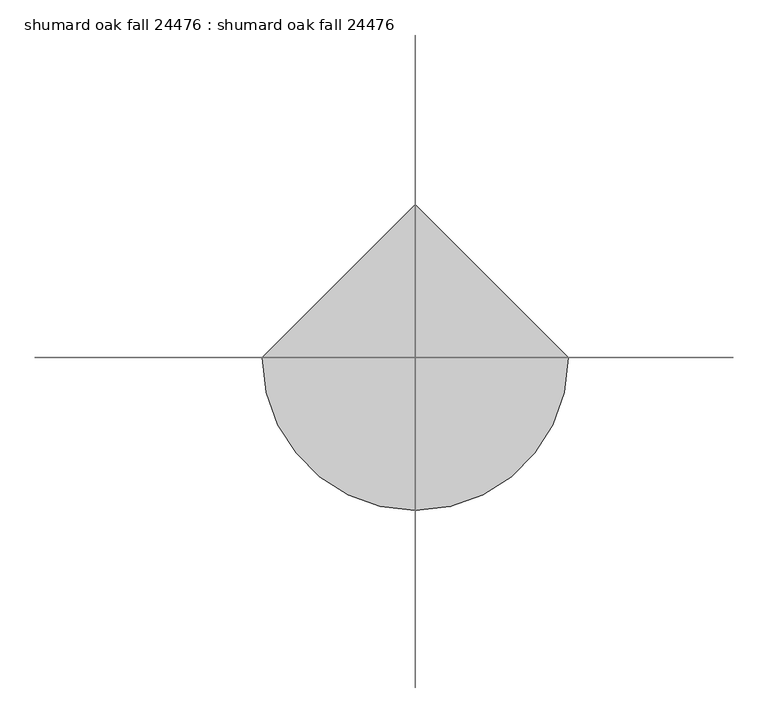
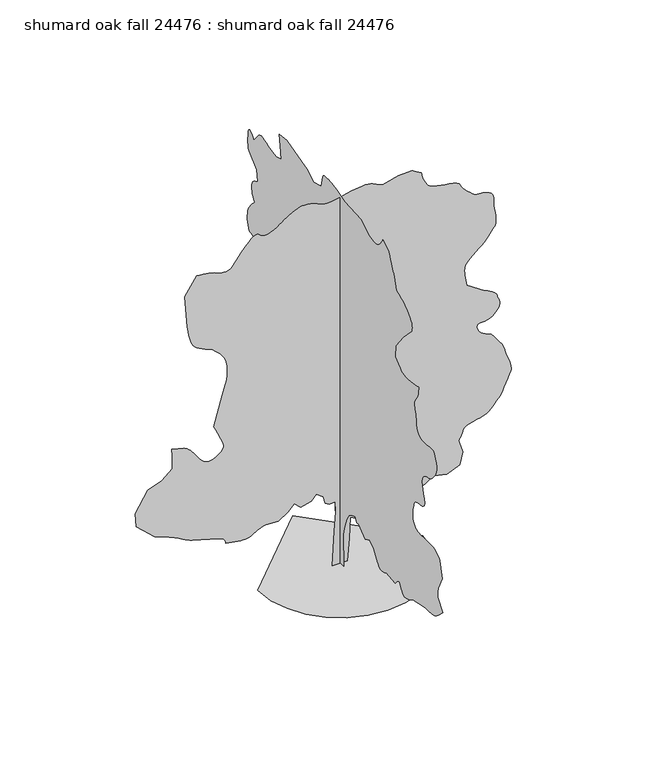
"""IFC4 building model written with IfcOpenShell, lengths in millimetres: proxy geometry, shumard oak fall 24476 : shumard oak fall 24476."""

from ifc_helpers import new_model, si_unit, origin, place, context, project, spatial, triangles, source, transform, mapped, element, save


def shumard_oak_fall_24476_shumard_oak_fall_24476_f3c00e57(model_context):
    return source(origin(), model_context, "Body", "Tessellation", [
        triangles([(-0.002261, 219.4990839, 0.0114695), (-0.002261, -202.1468545, 0.0114695), (-0.002261, -165.4815053, 1044.9594), (-0.002261, -238.8111863, 1356.611816), (-0.002261, -348.8074883, 1649.9305401), (-0.002261, -477.1331583, 1851.5859638), (-0.002261, -623.7925203, 1943.2492641), (-0.002261, -807.1167229, 2016.5789452), (-0.002261, -880.4464039, 1851.5859638), (-0.002261, -1008.7746174, 1888.2507317), (-0.002261, -1155.4339794, 1741.5913696), (-0.002261, -1357.0894032, 1613.2657722), (-0.002261, -1595.4095947, 1723.2602211), (-0.002261, -1815.3986378, 1576.6008591), (-0.002261, -1962.0604706, 1319.9470482), (-0.002261, -1997.5492928, 1269.2765945), (-0.002261, -2033.8382114, 1221.0141335), (-0.002261, -2071.73241, 1177.5624252), (-0.002261, -2112.0319851, 1141.3243029), (-0.002261, -2155.5370331, 1114.7076862), (-0.002261, -2203.0527374, 1100.1179518), (-0.002261, -2255.3767239, 1099.955389), (-0.002261, -2305.5645035, 1108.8834778), (-0.002261, -2347.093364, 1119.7317982), (-0.002261, -2381.4062405, 1132.1853985), (-0.002261, -2409.948103, 1145.9216967), (-0.002261, -2434.1594158, 1160.6206541), (-0.002261, -2455.4852943, 1175.9596888), (-0.002261, -2475.3657669, 1191.618762), (-0.002261, -2952.0087662, 1136.622773), (-0.002261, -2998.9986305, 1190.8694618), (-0.002261, -3044.9978577, 1240.6280525), (-0.002261, -3089.0922592, 1281.4101562), (-0.002261, -3130.3164871, 1308.7227333), (-0.002261, -3167.6796135, 1318.0750694), (-0.002261, -3200.2171623, 1304.9813919), (-0.002261, -3226.9884933, 1264.9485157), (-0.002261, -3253.8871422, 1207.3845148), (-0.002261, -3287.1865631, 1147.8978115), (-0.002261, -3326.5565437, 1091.299086), (-0.002261, -3371.7430298, 1042.3940042), (-0.002261, -3422.3396507, 1005.9958626), (-0.002261, -3478.092643, 986.9154139), (-0.002261, -3538.6462143, 989.9608675), (-0.002261, -3599.3521019, 1007.8145016), (-0.002261, -3656.2224678, 1029.5136858), (-0.002261, -3709.8927383, 1054.4208864), (-0.002261, -3760.9974678, 1081.8909393), (-0.002261, -3810.1717918, 1111.2888542), (-0.002261, -3858.0505554, 1141.9669235), (-0.002261, -3905.294474, 1173.2876135), (-0.002261, -4565.2617485, 1301.6132835), (-0.002261, -4647.5828865, 1301.7733028), (-0.002261, -4728.7613617, 1302.8960541), (-0.002261, -4807.7042175, 1305.9439785), (-0.002261, -4883.2693726, 1311.8748665), (-0.002261, -4954.3638702, 1321.6563915), (-0.002261, -5019.8447571, 1336.2461987), (-0.002261, -5078.5696609, 1356.611816), (-0.002261, -5135.1603928, 1386.0605999), (-0.002261, -5194.6474594, 1426.09086), (-0.002261, -5256.5471695, 1474.9426746), (-0.002261, -5320.3769943, 1530.8479832), (-0.002261, -5385.6294067, 1592.0465733), (-0.002261, -5451.8474579, 1656.7708202), (-0.002261, -5518.5474564, 1723.2602211), (-0.002261, -5261.9061447, 2016.5789452), (-0.002261, -5254.2612625, 2071.5216671), (-0.002261, -5247.8854889, 2126.1442051), (-0.002261, -5244.1008362, 2180.1268112), (-0.002261, -5244.1519958, 2233.1466854), (-0.002261, -5249.3336563, 2284.8837891), (-0.002261, -5260.9410873, 2335.0182289), (-0.002261, -5280.2195618, 2383.2273502), (-0.002261, -5481.8956238, 2804.8665848), (-0.002261, -5353.5493881, 3318.1744972), (-0.002261, -5343.5162796, 3332.34776), (-0.002261, -5313.5698517, 3368.644091), (-0.002261, -5264.0908951, 3417.7422569), (-0.002261, -5195.3584625, 3470.3963104), (-0.002261, -5107.7033478, 3517.2594383), (-0.002261, -5001.4551819, 3549.0601135), (-0.002261, -4876.9191788, 3556.5023918), (-0.002261, -4738.1593346, 3550.7364647), (-0.002261, -4595.2590454, 3548.4758469), (-0.002261, -4457.4642586, 3548.8060593), (-0.002261, -4334.0967888, 3550.7364647), (-0.002261, -4234.4781601, 3553.3020058), (-0.002261, -4167.8793182, 3555.5370438), (-0.002261, -4143.6223686, 3556.5023918), (-0.002261, -4129.3985275, 3566.1797081), (-0.002261, -4092.7461136, 3593.4847275), (-0.002261, -4042.6067322, 3635.877198), (-0.002261, -3987.9714043, 3690.7665802), (-0.002261, -3937.857312, 3755.5873329), (-0.002261, -3901.1798996, 3827.7992043), (-0.002261, -3886.9557678, 3904.8119453), (-0.002261, -3889.6480453, 3981.7738174), (-0.002261, -3897.1159035, 4055.8655159), (-0.002261, -3908.5965981, 4127.5442802), (-0.002261, -3923.3032585, 4197.2923485), (-0.002261, -3940.4225624, 4265.5928307), (-0.002261, -3959.1170609, 4332.9282555), (-0.002261, -3978.6243004, 4399.7808609), (-0.002261, -3994.6515198, 4419.3642586), (-0.002261, -4012.6094353, 4438.4398384), (-0.002261, -4034.4278709, 4456.5497795), (-0.002261, -4062.0122337, 4473.2377144), (-0.002261, -4097.2673492, 4487.969664), (-0.002261, -4142.1744919, 4500.3392578), (-0.002261, -4198.6131981, 4509.7880997), (-0.002261, -4266.863102, 4515.5540268), (-0.002261, -4340.573719, 4522.2850113), (-0.002261, -4411.7190857, 4537.6773857), (-0.002261, -4472.2723663, 4569.4271919), (-0.002261, -4514.2331772, 4625.2310532), (-0.002261, -4529.5493935, 4712.7847206), (-0.002261, -4510.270919, 4839.758947), (-0.002261, -4470.7739113, 4983.3196609), (-0.002261, -4434.4772896, 5115.0185989), (-0.002261, -4406.8420578, 5234.2206253), (-0.002261, -4393.3295105, 5340.2397354), (-0.002261, -4399.3744904, 5432.492244), (-0.002261, -4430.4132935, 5510.3177261), (-0.002261, -4491.9319221, 5573.0557571), (-0.002261, -4567.3444702, 5616.9978424), (-0.002261, -4637.3213036, 5643.9473602), (-0.002261, -4703.1074043, 5661.5747726), (-0.002261, -4766.0230408, 5677.6022827), (-0.002261, -4827.313195, 5699.725351), (-0.002261, -4888.2981354, 5735.6661804), (-0.002261, -4950.2490051, 5793.0446548), (-0.002261, -5013.3678268, 5866.0698486), (-0.002261, -5073.5908951, 5943.8953308), (-0.002261, -5125.8132889, 6026.8263153), (-0.002261, -5164.8783463, 6115.2435928), (-0.002261, -5185.6811462, 6209.4012177), (-0.002261, -5183.0650269, 6309.6799805), (-0.002261, -5151.8989059, 6416.3600967), (-0.002261, -5114.282016, 6517.2737045), (-0.002261, -5088.8312439, 6599.5698441), (-0.002261, -5065.3105865, 6662.6380875), (-0.002261, -5033.4590424, 6705.8180099), (-0.002261, -4983.0150284, 6728.499765), (-0.002261, -4903.6908005, 6729.9985107), (-0.002261, -4785.2506462, 6709.6788208), (-0.002261, -4644.7382927, 6687.2249588), (-0.002261, -4509.6866524, 6682.729303), (-0.002261, -4385.5061508, 6696.2168518), (-0.002261, -4277.7086609, 6727.6364456), (-0.002261, -4191.7298973, 6777.0142456), (-0.002261, -4132.9797043, 6844.3746689), (-0.002261, -4106.9449562, 6929.6677185), (-0.002261, -4098.029512, 7020.7516937), (-0.002261, -4087.1836624, 7106.0447433), (-0.002261, -4074.7123306, 7186.5375046), (-0.002261, -4060.9963074, 7263.169455), (-0.002261, -4046.2896469, 7336.9306503), (-0.002261, -4030.9481415, 7408.761731), (-0.002261, -4015.3017128, 7479.6277542), (-0.002261, -4000.0616547, 7530.732193), (-0.002261, -3987.71735, 7581.9895294), (-0.002261, -3981.1389725, 7633.5764969), (-0.002261, -3983.2216942, 7685.6215759), (-0.002261, -3996.8612686, 7738.3264984), (-0.002261, -4024.9028709, 7791.8185822), (-0.002261, -4070.2925423, 7846.2763046), (-0.002261, -4118.8067322, 7913.1036209), (-0.002261, -4155.4841446, 7996.8979248), (-0.002261, -4181.8746849, 8087.7534256), (-0.002261, -4199.6294151, 8175.7387527), (-0.002261, -4210.3226578, 8250.8719574), (-0.002261, -4215.5551872, 8303.2722473), (-0.002261, -4216.952195, 8322.9315125), (-0.002261, -4189.9012299, 8316.8865326), (-0.002261, -4117.3332756, 8301.5450272), (-0.002261, -4012.0251686, 8281.0724396), (-0.002261, -3886.8543205, 8259.6603745), (-0.002261, -3754.6219849, 8241.4231155), (-0.002261, -3628.1808655, 8230.5772659), (-0.002261, -3520.3075081, 8231.2632706), (-0.002261, -3429.2485313, 8247.1384644), (-0.002261, -3343.9301926, 8277.4401031), (-0.002261, -3263.437722, 8319.7822861), (-0.002261, -3186.8057716, 8371.7250458), (-0.002261, -3113.0442856, 8430.9068985), (-0.002261, -3041.213205, 8494.8640411), (-0.002261, -2970.3474724, 8561.259407), (-0.002261, -2988.6861786, 8946.2469543), (-0.002261, -3391.9868523, 9459.5545761), (-0.002261, -3850.3036446, 9936.1842041), (-0.002261, -3857.4662888, 9995.2898987), (-0.002261, -3860.4634895, 10055.5385468), (-0.002261, -3855.1042236, 10118.0231049), (-0.002261, -3837.2480461, 10183.8597839), (-0.002261, -3802.7295135, 10254.1927002), (-0.002261, -3747.3576027, 10330.1380646), (-0.002261, -3666.9668701, 10412.8399933), (-0.002261, -3572.6822182, 10492.2909576), (-0.002261, -3478.4228554, 10559.2705902), (-0.002261, -3384.1382034, 10615.8113251), (-0.002261, -3289.8535515, 10664.0200104), (-0.002261, -3195.5688995, 10705.9814026), (-0.002261, -3101.2842476, 10743.77677), (-0.002261, -3006.9995956, 10779.4629639), (-0.002261, -2979.491391, 10873.4944336), (-0.002261, -2951.8055809, 10965.8992584), (-0.002261, -2923.7892677, 11055.1042786), (-0.002261, -2895.2904259, 11139.5072662), (-0.002261, -2866.1823189, 11217.4862274), (-0.002261, -2836.2356003, 11287.4366089), (-0.002261, -2805.3494041, 11347.7875763), (-0.002261, -2771.0846352, 11413.5730957), (-0.002261, -2733.3151382, 11494.7518616), (-0.002261, -2695.1895584, 11582.0511841), (-0.002261, -2659.9853119, 11666.1251221), (-0.002261, -2630.8516251, 11737.6765686), (-0.002261, -2611.0141731, 11787.4351593), (-0.002261, -2603.698922, 11806.1037872), (-0.002261, -2292.0441078, 11989.4158539), (-0.002261, -2276.0623798, 11957.8177826), (-0.002261, -2258.4779881, 11925.2813965), (-0.002261, -2237.6856525, 11890.8137329), (-0.002261, -2212.0850349, 11853.4497345), (-0.002261, -2180.0708553, 11812.2255066), (-0.002261, -2140.0379791, 11766.2259888), (-0.002261, -2090.3862133, 11714.4361267), (-0.002261, -2030.5793987, 11669.5795624), (-0.002261, -1962.1138103, 11643.0369965), (-0.002261, -1886.4320927, 11631.6830383), (-0.002261, -1804.9770355, 11632.5469391), (-0.002261, -1719.1937542, 11642.5544678), (-0.002261, -1630.5250385, 11658.6325562), (-0.002261, -1540.413533, 11677.7581329), (-0.002261, -1137.1002874, 11952.7378601), (-0.002261, -257.1441153, 12007.7542694), (-0.002261, -143.4615103, 12039.0221283), (-0.002261, -31.2221381, 12069.3237671), (-0.002261, 78.1307869, 12097.6952911), (-0.002261, 183.1547906, 12123.1972229), (-0.002261, 282.4069083, 12144.8377625), (-0.002261, 374.4436778, 12161.678595), (-0.002261, 457.8190392, 12172.7523376), (-0.002261, 540.0209258, 12181.1855438), (-0.002261, 626.0734131, 12188.6781097), (-0.002261, 710.8406954, 12191.9802338), (-0.002261, 789.1944883, 12187.9165283), (-0.002261, 856.001457, 12173.286026), (-0.002261, 906.1358969, 12144.8377625), (-0.002261, 934.464473, 12099.3975128), (-0.002261, 1026.1253025, 11732.7745422), (-0.002261, 1429.4386208, 11622.7673035), (-0.002261, 1796.0870258, 11842.7562012), (-0.002261, 2254.3987312, 11952.7378601), (-0.002261, 2859.3748856, 12136.0755066), (-0.002261, 3262.6755592, 12081.0846771), (-0.002261, 3226.023436, 11732.7745422), (-0.002261, 3152.6939003, 11329.4491608), (-0.002261, 3446.0126244, 11237.7803375), (-0.002261, 3739.3313484, 11292.771167), (-0.002261, 3852.7421585, 11335.3918213), (-0.002261, 3963.1048988, 11374.2801453), (-0.002261, 4067.3717903, 11405.8258942), (-0.002261, 4162.5200523, 11426.2990631), (-0.002261, 4245.476326, 11432.0138306), (-0.002261, 4313.1925415, 11419.2878632), (-0.002261, 4362.6209198, 11384.4399902), (-0.002261, 4637.600647, 11054.4682709), (-0.002261, 4700.0846237, 11127.5184631), (-0.002261, 4760.3332718, 11191.1203949), (-0.002261, 4816.0609749, 11235.7990631), (-0.002261, 4865.082692, 11252.1062073), (-0.002261, 4905.1133881, 11230.5668243), (-0.002261, 4933.9168625, 11161.7326538), (-0.002261, 4949.2583679, 11036.1298553), (-0.002261, 4953.90634, 10896.6337189), (-0.002261, 4952.7889664, 10788.8868073), (-0.002261, 4946.870723, 10707.5813049), (-0.002261, 4937.0660889, 10647.4593933), (-0.002261, 4924.416861, 10603.2132568), (-0.002261, 4909.8119385, 10569.5327545), (-0.002261, 4894.2675385, 10541.1612305), (-0.002261, 4472.6281586, 10192.8255157), (-0.002261, 4435.9504555, 9807.8641296), (-0.002261, 4494.5989105, 9783.9632629), (-0.002261, 4551.4439873, 9758.1566986), (-0.002261, 4604.7840454, 9728.4893234), (-0.002261, 4652.8407051, 9693.0560211), (-0.002261, 4693.8361679, 9649.9272583), (-0.002261, 4726.0179245, 9597.1711761), (-0.002261, 4747.6078857, 9532.8588226), (-0.002261, 4755.837616, 9462.1706955), (-0.002261, 4750.6050865, 9391.4569885), (-0.002261, 4734.1459167, 9320.7438629), (-0.002261, 4708.6951447, 9250.0301559), (-0.002261, 4676.5133881, 9179.316449), (-0.002261, 4639.8612648, 9108.6033234), (-0.002261, 4600.9485237, 9037.8896164), (-0.002261, 4659.6225586, 8978.9362381), (-0.002261, 4716.8740059, 8919.8305435), (-0.002261, 4771.2299904, 8860.3946365), (-0.002261, 4821.2679245, 8800.4762009), (-0.002261, 4865.5146423, 8739.9229202), (-0.002261, 4902.547847, 8678.581897), (-0.002261, 4930.919371, 8616.2502365), (-0.002261, 4951.2902206, 8555.5446396), (-0.002261, 4965.8951431, 8498.6742737), (-0.002261, 4975.6741974, 8445.0037125), (-0.002261, 4981.5924408, 8393.8992737), (-0.002261, 4984.6405106, 8344.7249496), (-0.002261, 4985.7578842, 8296.8458954), (-0.002261, 4985.9357803, 8249.6022675), (-0.002261, 4875.9285416, 7937.9445465), (-0.002261, 4824.8999702, 7929.765976), (-0.002261, 4773.9984261, 7919.6817078), (-0.002261, 4723.4526741, 7905.7122116), (-0.002261, 4673.363871, 7886.0017868), (-0.002261, 4623.9354927, 7858.5697403), (-0.002261, 4575.2945663, 7821.5365356), (-0.002261, 4527.618988, 7772.9464783), (-0.002261, 4484.2103004, 7715.2883698), (-0.002261, 4447.5581772, 7652.804393), (-0.002261, 4416.4940849, 7586.332869), (-0.002261, 4389.9256485, 7516.635379), (-0.002261, 4366.7354942, 7444.5246643), (-0.002261, 4345.7806686, 7370.8140472), (-0.002261, 4325.9687965, 7296.3162689), (-0.002261, 4283.0426376, 7237.3628906), (-0.002261, 4241.8948586, 7178.257196), (-0.002261, 4204.2520981, 7118.8212891), (-0.002261, 4171.9180252, 7058.9028534), (-0.002261, 4146.6448586, 6998.3489914), (-0.002261, 4130.1856888, 6936.9829697), (-0.002261, 4124.2930252, 6874.676889), (-0.002261, 4142.6317314, 6379.682103), (-0.002261, 4185.5575996, 6375.3643433), (-0.002261, 4226.7056694, 6368.6333588), (-0.002261, 4264.3484299, 6357.076506), (-0.002261, 4296.6825027, 6338.3311386), (-0.002261, 4321.9553787, 6309.9340347), (-0.002261, 4338.4145485, 6269.5481277), (-0.002261, 4344.2819229, 6214.7096146), (-0.002261, 4342.6817299, 6151.3111588), (-0.002261, 4338.2113632, 6086.9732254), (-0.002261, 4331.3027733, 6021.822551), (-0.002261, 4322.4887764, 5956.0108704), (-0.002261, 4312.2271935, 5889.7428223), (-0.002261, 4301.0005531, 5823.1439804), (-0.002261, 4289.2910934, 5756.3928223), (-0.002261, 4270.9523872, 5389.7442719), (-0.002261, 4619.2875206, 5408.0832687), (-0.002261, 5004.2491974, 5481.4130951), (-0.002261, 5086.1895447, 5453.6758347), (-0.002261, 5164.7516098, 5424.4915695), (-0.002261, 5236.6082703, 5392.4115509), (-0.002261, 5298.3300842, 5356.0131912), (-0.002261, 5346.5899292, 5313.8494858), (-0.002261, 5378.009523, 5264.4716858), (-0.002261, 5389.2361633, 5206.4072067), (-0.002261, 5386.0357773, 5132.8744858), (-0.002261, 5377.0444656, 5040.0882889), (-0.002261, 5363.2778641, 4931.2751633), (-0.002261, 5345.6248718, 4809.634623), (-0.002261, 5325.1017059, 4678.3676353), (-0.002261, 5302.6478439, 4540.6745865), (-0.002261, 5279.2545044, 4399.7808609), (-0.002261, 5114.2564362, 3959.8027748), (-0.002261, 5024.1375183, 3909.2570229), (-0.002261, 4935.4661865, 3861.7337608), (-0.002261, 4849.6903175, 3820.3063477), (-0.002261, 4768.2327896, 3788.0228531), (-0.002261, 4692.5661873, 3767.9316376), (-0.002261, 4624.0880997, 3763.0801895), (-0.002261, 4564.2711113, 3776.4912895), (-0.002261, 4050.9631989, 3996.4804779), (-0.002261, 3537.6555771, 3831.4824097), (-0.002261, 3171.0070267, 3574.841098), (-0.002261, 2804.3587669, 3024.8557732), (-0.002261, 2768.8748863, 2970.1951561), (-0.002261, 2732.6038445, 2917.4393646), (-0.002261, 2694.7070297, 2868.5190948), (-0.002261, 2654.3972809, 2825.3897507), (-0.002261, 2610.887146, 2789.9570297), (-0.002261, 2563.3891731, 2764.1504654), (-0.002261, 2511.0525421, 2749.8757553), (-0.002261, 2458.8327644, 2745.1260452), (-0.002261, 2409.8236919, 2745.4815468), (-0.002261, 2360.4918194, 2749.3932266), (-0.002261, 2307.3119259, 2755.2097321), (-0.002261, 2246.7558838, 2761.3564499), (-0.002261, 2175.2957108, 2766.2334778), (-0.002261, 2089.4057499, 2768.2144615), (-0.002261, 1997.2622463, 2761.2550026), (-0.002261, 1908.966909, 2741.798632), (-0.002261, 1823.8796608, 2711.9283623), (-0.002261, 1741.357663, 2673.7013351), (-0.002261, 1660.7585129, 2629.251432), (-0.002261, 1581.4421333, 2580.6105057), (-0.002261, 1502.7683018, 2529.8868576), (-0.002261, 1392.7737076, 2218.2343689), (-0.002261, 1081.123835, 1869.9195831), (-0.002261, 1038.0988449, 1823.313271), (-0.002261, 988.3377834, 1777.6695454), (-0.002261, 932.9658726, 1732.8259163), (-0.002261, 873.1057909, 1688.6248352), (-0.002261, 809.8776735, 1644.9064281), (-0.002261, 744.404199, 1601.5055889), (-0.002261, 677.8105894, 1558.2672398), (-0.002261, 567.8161042, 1943.2492641), (-0.002261, 384.4893582, 2199.9032204), (-0.002261, 311.1621843, 2034.9100937), (-0.002261, 256.16367, 1778.2562828), (-0.002261, 237.8317585, 1319.9470482), (-0.002261, 201.1664093, 678.3109949), (227.1495435, 0.0005814, 0.0290322), (-249.4926201, 0.0005814, 0.0290322), (-176.1637021, 0.0005159, 1099.9731932), (-139.4986073, 0.0004774, 1741.6091011), (-157.8310275, 0.0004578, 2071.5927383), (-341.1570105, 0.0004589, 2053.2615898), (-469.4826805, 0.0004547, 2126.5912708), (-524.4786695, 0.0004403, 2364.9114624), (-744.470256, 0.0004316, 2511.5708244), (-891.1296181, 0.0004414, 2346.5778431), (-1221.1106392, 0.000447, 2254.9170135), (-1422.7685337, 0.0004361, 2438.2411434), (-1624.4239574, 0.000448, 2236.5832489), (-1917.7426815, 0.0004589, 2053.2615898), (-2357.7232384, 0.0004578, 2071.5927383), (-2577.7147522, 0.0004634, 1979.929438), (-2624.9586708, 0.0004655, 1944.816465), (-2672.8377251, 0.0004676, 1911.143811), (-2722.0120491, 0.0004694, 1880.3590622), (-2773.1167786, 0.0004708, 1853.9023922), (-2826.7867584, 0.0004722, 1833.219207), (-2883.6321259, 0.0004729, 1819.7496803), (-2944.3633026, 0.0004732, 1814.9389275), (-3012.0286491, 0.0004732, 1817.0776051), (-3088.3556763, 0.0004729, 1823.0618328), (-3171.8962166, 0.0004722, 1832.2566204), (-3261.2023933, 0.0004715, 1844.0141876), (-3354.8266205, 0.0004708, 1857.6972187), (-3451.3718903, 0.0004697, 1872.662875), (-3549.3394569, 0.000469, 1888.2686085), (-3553.8606926, 0.0004666, 1927.4454323), (-3562.115712, 0.0004641, 1965.9797081), (-3577.7112717, 0.000462, 2003.2338295), (-3604.3811554, 0.0004599, 2038.5626324), (-3645.8085686, 0.0004578, 2071.3260395), (-3705.6508461, 0.0004561, 2100.8815029), (-3787.6420624, 0.0004547, 2126.5912708), (-4594.2684082, 0.0004403, 2364.9114624), (-4660.1306671, 0.0004393, 2385.8106228), (-4730.463002, 0.0004375, 2415.3659409), (-4803.0306656, 0.0004354, 2451.0149277), (-4875.623909, 0.000433, 2490.1916061), (-4945.9562439, 0.0004305, 2530.3313072), (-5011.8185028, 0.0004284, 2568.8757568), (-5070.9241974, 0.0004263, 2603.2419731), (-5134.4749695, 0.0004242, 2636.2617599), (-5213.4178253, 0.0004221, 2672.1773003), (-5305.1878052, 0.0004197, 2710.5057747), (-5407.219368, 0.0004176, 2750.7393654), (-5516.947554, 0.0004151, 2792.446122), (-5631.8062408, 0.0004123, 2835.0926468), (-5749.2298874, 0.0004099, 2878.2217003), (-6317.52892, 0.000378, 3409.8683189), (-6354.1807526, 0.0003518, 3849.846405), (-5969.2187851, 0.0003147, 4473.1359764), (-5529.2409897, 0.0003049, 4638.1340446), (-5199.2448532, 0.0002884, 4913.1140625), (-5199.2448532, 0.0002636, 5334.7534424), (-5217.5832687, 0.0002503, 5554.7423401), (-4832.5963028, 0.0002559, 5463.099678), (-4789.264064, 0.0002576, 5435.1339432), (-4745.0935043, 0.0002594, 5404.4509323), (-4699.3480408, 0.0002615, 5368.3322067), (-4651.1896431, 0.0002639, 5324.0093307), (-4599.8311501, 0.0002674, 5268.8150253), (-4544.4592392, 0.0002716, 5199.9814362), (-4484.2867493, 0.0002765, 5114.7645447), (-4423.3012276, 0.0002818, 5025.254892), (-4364.5513252, 0.0002867, 4946.3120361), (-4305.8264214, 0.0002905, 4879.560878), (-4244.8411903, 0.0002937, 4826.5766121), (-4179.3600128, 0.0002961, 4789.0100098), (-4107.1481415, 0.0002972, 4768.4359749), (-4025.9696663, 0.0002972, 4766.4547005), (-3937.1968872, 0.0002961, 4786.7746811), (-3847.7889725, 0.0002937, 4827.9227509), (-3763.8167725, 0.0002902, 4883.8280594), (-3691.4014252, 0.0002863, 4948.3944672), (-3636.613781, 0.0002825, 5015.5269974), (-3605.5496887, 0.0002786, 5079.1283478), (-3604.3305771, 0.0002755, 5133.1029602), (-3625.9205383, 0.000272, 5191.4720718), (-3658.1020042, 0.0002674, 5270.034137), (-3699.0977577, 0.0002615, 5365.4364532), (-3747.1291283, 0.0002552, 5474.3263184), (-3800.4688957, 0.0002482, 5593.2998703), (-3857.3395523, 0.0002405, 5719.0038254), (-3915.9880074, 0.0002328, 5848.0610641), (-3659.3214066, 0.0001771, 6783.0336456), (-3624.2186073, 0.0001708, 6888.8498611), (-3590.5383957, 0.0001645, 6993.2440704), (-3559.7536469, 0.0001586, 7094.7419449), (-3533.2866577, 0.0001526, 7191.8970612), (-3512.6111755, 0.0001474, 7283.2856689), (-3499.1492065, 0.0001421, 7367.4613449), (-3494.3233383, 0.0001379, 7443.0009201), (-3495.5677391, 0.0001334, 7516.6859573), (-3499.6826042, 0.0001288, 7594.8928116), (-3507.3280678, 0.0001239, 7675.3344131), (-3519.1389748, 0.000119, 7755.7760147), (-3535.7504608, 0.0001145, 7833.9572891), (-3557.8232414, 0.0001099, 7907.6679062), (-3585.9915802, 0.0001061, 7974.6219589), (-3622.2373329, 0.0001022, 8036.9536194), (-3667.1191864, 9.87e-05, 8098.3196411), (-3719.2398422, 9.52e-05, 8158.8735031), (-3777.1264252, 9.14e-05, 8218.7919388), (-3839.3307678, 8.79e-05, 8278.2022659), (-3904.430864, 8.44e-05, 8337.3335403), (-3970.9788368, 8.09e-05, 8396.2869186), (-4076.5918671, 7.84e-05, 8439.5685791), (-4179.4617508, 7.56e-05, 8483.3321869), (-4276.8959198, 7.32e-05, 8528.0870132), (-4366.1768074, 7.04e-05, 8574.2644272), (-4444.5103981, 6.76e-05, 8622.3719559), (-4509.254702, 6.44e-05, 8672.8671295), (-4557.6162849, 6.13e-05, 8726.2574753), (-4595.665416, 5.71e-05, 8797.4537109), (-4630.8443733, 5.15e-05, 8893.9734009), (-4662.4674431, 4.48e-05, 9005.2509109), (-4689.9500679, 3.78e-05, 9120.6938644), (-4712.6068245, 3.12e-05, 9229.7354645), (-4729.828157, 2.59e-05, 9321.7594986), (-4740.9277702, 2.21e-05, 9386.2247498), (-4814.2575966, -3.92e-05, 10412.8399933), (-4447.6090462, -7.32e-05, 10981.1390259), (-4349.6414795, -7.25e-05, 10969.2269623), (-4253.1214989, -7.18e-05, 10956.5009949), (-4159.4719826, -7.07e-05, 10942.1751251), (-4070.1658058, -6.97e-05, 10925.4621918), (-3986.6252655, -6.86e-05, 10905.5238739), (-3910.3238182, -6.72e-05, 10881.5706848), (-3842.658181, -6.55e-05, 10852.8189514), (-3773.849881, -6.37e-05, 10825.0311127), (-3696.4051895, -6.27e-05, 10805.5741608), (-3615.1255577, -6.2e-05, 10796.0491608), (-3534.7854034, -6.23e-05, 10798.0815948), (-3460.2364655, -6.3e-05, 10813.2702026), (-3396.2540337, -6.48e-05, 10843.1916321), (-3347.6639763, -6.76e-05, 10889.4957825), (-3054.3452522, -9.07e-05, 11274.4583313), (-2976.0116615, -9.59e-05, 11364.1447174), (-2898.9227623, -0.0001012, 11449.8185577), (-2824.4246933, -0.0001057, 11527.4917236), (-2753.7618553, -0.0001096, 11593.1260895), (-2688.2300995, -0.0001127, 11642.7312012), (-2629.1244049, -0.0001145, 11672.2724213), (-2577.7147522, -0.0001148, 11677.7837128), (-2536.3434402, -0.0001138, 11663.9915314), (-2502.6707863, -0.0001124, 11641.5382507), (-2470.9233055, -0.000111, 11615.2491577), (-2435.3278038, -0.0001096, 11589.9251221), (-2390.1107964, -0.0001082, 11570.3414337), (-2329.5038853, -0.0001078, 11561.3757019), (-2247.7287895, -0.0001082, 11567.776474), (-2150.0253056, -0.0001099, 11595.5898926), (-2049.7588966, -0.0001124, 11641.9696198), (-1953.3381832, -0.0001159, 11698.6370911), (-1867.1815235, -0.0001194, 11757.2090973), (-1797.6998634, -0.0001225, 11809.3803314), (-1751.3093811, -0.0001246, 11846.7699097), (-1734.4184063, -0.0001257, 11861.0957794), (-1713.7352211, -0.0001264, 11874.3542725), (-1658.7366886, -0.0001285, 11908.7707764), (-1580.0095173, -0.0001313, 11956.3446167), (-1488.1328579, -0.0001344, 12009.0495392), (-1393.6932735, -0.0001372, 12058.8592896), (-1307.269915, -0.0001397, 12097.7720306), (-1239.4444038, -0.0001407, 12117.7615082), (-1175.0935352, -0.0001411, 12122.2065857), (-1095.0303263, -0.0001411, 12119.5648865), (-1003.7428751, -0.0001404, 12109.5829376), (-905.7193525, -0.0001393, 12091.8793671), (-805.4530163, -0.0001379, 12066.1739594), (-707.4294937, -0.0001358, 12032.1388275), (-616.1420425, -0.0001334, 11989.4414337), (-519.0278395, -0.0001313, 11954.5923981), (-402.6731684, -0.0001306, 11941.8675934), (-270.2835022, -0.0001306, 11947.5823608), (-125.0678747, -0.000132, 11968.0543671), (29.7687521, -0.0001337, 11999.5756989), (191.019118, -0.0001362, 12038.4884399), (355.4775026, -0.0001386, 12081.0846771), (468.9975357, -0.0001397, 12096.4767609), (580.1147358, -0.0001404, 12109.9643097), (686.421183, -0.0001411, 12119.5648865), (785.5140444, -0.0001411, 12123.4262787), (874.9828566, -0.0001411, 12119.5648865), (952.4298735, -0.00014, 12106.1029175), (1015.4446318, -0.0001386, 12081.0846771), (1068.3019432, -0.0001369, 12051.7980927), (1117.3137045, -0.0001355, 12026.3729004), (1163.1174494, -0.0001341, 12004.121933), (1206.358342, -0.000133, 11984.4626678), (1247.6713726, -0.000132, 11966.7079376), (1287.7042488, -0.0001309, 11950.2496399), (1327.094577, -0.0001299, 11934.4250244), (1803.737431, -0.0001376, 12062.7706787), (2225.3843685, -0.0001386, 12081.0846771), (2518.7032379, -0.0001288, 11916.111026), (2522.9244919, -0.0001264, 11872.7032104), (2528.9113358, -0.0001236, 11828.1768585), (2538.4235458, -0.0001208, 11781.4157593), (2553.2293282, -0.000118, 11731.2757965), (2575.0986328, -0.0001145, 11676.6663391), (2605.7563545, -0.000111, 11616.417691), (2647.0314514, -0.0001071, 11549.4636383), (2688.5094429, -0.0001033, 11488.1476135), (2722.9265282, -0.0001008, 11442.88526), (2756.7084778, -9.87e-05, 11409.4838104), (2796.2560638, -9.7e-05, 11383.7795654), (2847.995929, -9.59e-05, 11361.5797577), (2918.3282639, -9.45e-05, 11338.7706848), (3013.6797112, -9.28e-05, 11311.1351624), (3131.2053864, -9.14e-05, 11284.5158569), (3258.0272964, -9e-05, 11264.3229034), (3385.509922, -8.89e-05, 11245.7054352), (3504.965712, -8.75e-05, 11223.9114166), (3607.7341484, -8.58e-05, 11194.0923065), (3685.1785492, -8.33e-05, 11151.4204926), (3728.6378151, -7.98e-05, 11091.1462646), (3760.7687027, -7.56e-05, 11020.9656647), (3808.2919647, -7.14e-05, 10951.7512848), (3868.6170616, -6.72e-05, 10883.349646), (3939.2290306, -6.34e-05, 10815.5572723), (4017.5370415, -5.92e-05, 10748.2718445), (4100.9505547, -5.53e-05, 10681.3177917), (4186.9546074, -5.11e-05, 10614.4904755), (4307.9094337, -5.04e-05, 10602.0958832), (4423.8854942, -4.97e-05, 10586.0177948), (4529.9304749, -4.83e-05, 10562.5471344), (4621.0400299, -4.62e-05, 10528.0294739), (4692.2868439, -4.31e-05, 10478.7534119), (4738.6927322, -3.92e-05, 10411.036615), (4755.2533493, -3.4e-05, 10321.1723328), (4756.3201447, -2.84e-05, 10227.5989746), (4759.3173454, -2.35e-05, 10149.3921204), (4763.9147392, -1.96e-05, 10084.03797), (4769.8076935, -1.65e-05, 10028.9448212), (4776.6401253, -1.37e-05, 9981.5232971), (4784.1076927, -1.09e-05, 9939.2584351), (4791.9310524, -8.8e-06, 9899.5329529), (4807.2725578, -3.2e-06, 9805.5782227), (4820.3534454, 2.5e-06, 9713.5286087), (4828.9639664, 7.7e-06, 9625.3398056), (4830.8437935, 1.26e-05, 9542.9425095), (4823.7317276, 1.72e-05, 9468.2156754), (4805.3930214, 2.1e-05, 9403.1155792), (4773.5920555, 2.42e-05, 9349.5729172), (4733.0285431, 2.73e-05, 9298.2138428), (4689.2387741, 3.08e-05, 9239.4639404), (4641.3091415, 3.47e-05, 9174.948111), (4588.2231377, 3.85e-05, 9106.2662567), (4529.0668648, 4.27e-05, 9035.0194427), (4462.8491043, 4.73e-05, 8962.8075714), (4388.6050896, 5.15e-05, 8891.2555435), (4302.3975609, 5.6e-05, 8817.4437698), (4206.2586617, 6.06e-05, 8738.5003326), (4108.1640678, 6.55e-05, 8656.0268784), (4016.1909027, 7.04e-05, 8571.6483078), (3938.3145515, 7.56e-05, 8486.913945), (3882.5615593, 8.05e-05, 8403.5004318), (3856.9584709, 8.54e-05, 8322.9570923), (3852.8436058, 9e-05, 8243.302652), (3855.485305, 9.49e-05, 8161.7436768), (3863.7147446, 9.98e-05, 8078.5842178), (3876.4148415, 0.000105, 7994.1294891), (3892.5185097, 0.0001099, 7908.7347015), (3910.831636, 0.0001152, 7822.6794891), (3930.2880066, 0.0001204, 7736.3196442), (4480.2733315, 0.0001421, 7369.6710938), (4501.5839493, 0.0001428, 7360.1460938), (4556.6003586, 0.0001442, 7333.9587387), (4631.7841415, 0.0001467, 7294.6140472), (4713.7244888, 0.0001495, 7245.668779), (4788.9338516, 0.000153, 7190.60121), (4843.9246811, 0.0001561, 7132.9942612), (4865.2605881, 0.0001596, 7076.3523697), (4876.6907043, 0.0001628, 7022.8347061), (4902.8780594, 0.0001659, 6969.3426224), (4931.6309555, 0.0001694, 6911.3543015), (4950.7571136, 0.0001736, 6844.3746689), (4948.0898346, 0.0001782, 6763.9330673), (4911.438002, 0.0001841, 6665.5588394), (4828.5831757, 0.0001915, 6544.705751), (4714.3087555, 0.0001974, 6441.8614471), (4596.8339493, 0.0002006, 6388.7501541), (4484.1850113, 0.000202, 6367.6938812), (4384.3379082, 0.0002023, 6361.0640533), (4305.3438927, 0.000203, 6351.2344208), (4255.2045113, 0.0002048, 6320.5514099), (4241.9457275, 0.000209, 6251.387027), (4261.0210167, 0.0002139, 6165.12892), (4300.3148392, 0.0002181, 6093.2978394), (4356.423333, 0.0002219, 6033.4811417), (4426.0190849, 0.0002247, 5983.2906006), (4505.7241035, 0.0002272, 5940.3141541), (4592.1348175, 0.0002296, 5902.1629944), (4681.9238136, 0.0002317, 5866.400061), (4771.6616501, 0.0002384, 5752.8878036), (4857.7168625, 0.000245, 5641.7626099), (4936.3806656, 0.0002513, 5535.4638657), (5003.9951431, 0.0002573, 5436.3786346), (5056.8523819, 0.0002629, 5346.8945618), (5091.2694672, 0.0002674, 5269.4504517), (5103.5629028, 0.0002709, 5206.4327866), (5118.5491974, 0.0002755, 5131.0711075), (5155.9631927, 0.0002821, 5023.3247772), (5204.57883, 0.0002895, 4895.6895447), (5253.2194656, 0.0002975, 4760.689064), (5290.633461, 0.0003052, 4630.8190842), (5305.5941757, 0.0003122, 4518.5765167), (5286.899968, 0.0003171, 4436.4838531), (5243.4404114, 0.0003217, 4355.4071159), (5192.9452377, 0.0003283, 4245.7809586), (5137.2939835, 0.000336, 4119.4668663), (5078.4423431, 0.0003437, 3988.3777748), (5018.3210129, 0.0003511, 3864.3243004), (4958.8339462, 0.0003574, 3759.1940895), (4901.913002, 0.0003619, 3684.8483368), (4846.7186966, 0.0003654, 3625.9458275), (4790.2038322, 0.0003693, 3561.6076035), (4731.148716, 0.0003731, 3495.3136848), (4668.2586594, 0.000377, 3430.6455391), (4600.2119408, 0.0003805, 3371.1078941), (4525.7647408, 0.0003836, 3320.2319298), (4443.595919, 0.0003857, 3281.522374), (4346.4919624, 0.0003875, 3252.8203468), (4234.6304764, 0.0003892, 3227.0140732), (4117.9431221, 0.0003906, 3200.2424515), (4006.4118484, 0.0003924, 3168.6449615), (3909.9427368, 0.0003948, 3128.4113708), (3838.4671577, 0.000398, 3075.6555794), (3801.9676414, 0.0004022, 3006.5423561), (3782.4095329, 0.0004064, 2937.2768166), (3757.7209236, 0.0004095, 2883.4033607), (3731.7367538, 0.000412, 2840.121991), (3708.3431236, 0.0004144, 2802.5806778), (3691.325267, 0.0004165, 2766.0302925), (3684.5942825, 0.000419, 2725.6188057), (3691.9856918, 0.0004218, 2676.5715088), (3801.9676414, 0.0004428, 2328.2466946), (3710.2991089, 0.0004666, 1924.9333763), (3306.9984352, 0.0004764, 1759.9428658), (2903.6724724, 0.0004711, 1851.6036953), (2500.3694733, 0.0004862, 1594.9497391), (2207.0507492, 0.0004764, 1759.9428658), (1785.4038116, 0.0004655, 1943.2645248), (1757.7736668, 0.0004666, 1927.1787334), (1729.3384838, 0.0004676, 1908.8451141), (1699.3004917, 0.000469, 1886.0232513), (1666.859594, 0.0004708, 1856.4677879), (1631.2082817, 0.0004729, 1817.9310413), (1591.5512547, 0.000476, 1768.1724506), (1547.0836201, 0.0004799, 1704.9443333), (1500.4771626, 0.0004837, 1638.5081268), (1454.833437, 0.0004872, 1579.7707237), (1409.992424, 0.0004904, 1527.4468826), (1365.7913429, 0.0004932, 1480.2512169), (1322.0704651, 0.0004956, 1436.9061882), (1278.6720966, 0.0004981, 1396.1265553), (1235.4337475, 0.0005005, 1356.6295475), (1290.4296638, 0.0005236, 971.6475231), (1258.8423477, 0.0005243, 960.0499025), (1226.2922997, 0.0005247, 949.5724171), (1191.8194038, 0.0005254, 941.3428322), (1154.4611464, 0.0005257, 936.4787395), (1113.2522518, 0.0005257, 936.1053612), (1067.2326044, 0.0005254, 941.3428322), (1015.4446318, 0.0005247, 953.3138311), (961.5154381, 0.0005233, 973.3035994), (909.5115629, 0.0005219, 1000.9895548), (859.1104242, 0.0005198, 1035.0889996), (809.9919834, 0.0005173, 1074.3192358), (761.8362019, 0.0005149, 1117.3975657), (714.323041, 0.0005121, 1163.0412912), (667.1273752, 0.0005093, 1209.9677147), (318.8101187, 0.0004984, 1393.2944607), (282.1478216, 0.0005387, 714.9936396), (-2555.6678421, 0.0, 0.0), (-2488.1062683, -585.5910004, 0.0), (-2295.6864727, -1123.3614458, 0.0), (-1993.815509, -1597.90639, 0.0), (-1597.90639, -1993.815509, 0.0), (-1123.3614458, -2295.6838566, 0.0), (-585.5910004, -2488.1062683, 0.0), (0.0001117, -2555.6678421, 0.0), (585.5910004, -2488.1062683, 0.0), (1123.3614458, -2295.6864727, 0.0), (1597.90639, -1993.815509, 0.0), (1993.815509, -1597.90639, 0.0), (2295.6864727, -1123.3614458, 0.0), (2488.1062683, -585.5910004, 0.0), (2555.6678421, 0.0002233, 0.0), (-0.0003351, 2555.6678421, 0.0)], [[407, 408, 409], [173, 174, 175], [406, 407, 409], [219, 220, 221], [1, 2, 3], [414, 1, 3], [413, 414, 3], [413, 3, 4], [412, 413, 4], [412, 4, 5], [255, 256, 257], [219, 221, 222], [65, 66, 67], [405, 406, 409], [8, 9, 10], [219, 222, 223], [404, 405, 409], [64, 65, 67], [412, 5, 6], [411, 412, 6], [403, 404, 409], [219, 223, 224], [172, 173, 175], [172, 175, 176], [171, 172, 176], [171, 176, 177], [170, 171, 177], [254, 255, 257], [254, 257, 258], [402, 403, 409], [63, 64, 67], [218, 219, 224], [401, 402, 409], [218, 224, 225], [217, 218, 225], [312, 313, 314], [216, 217, 225], [216, 225, 226], [170, 177, 178], [169, 170, 178], [168, 169, 178], [167, 168, 178], [167, 178, 179], [166, 167, 179], [166, 179, 180], [165, 166, 180], [11, 12, 13], [216, 226, 227], [215, 216, 227], [400, 401, 409], [400, 409, 410], [399, 400, 410], [29, 30, 31], [62, 63, 67], [214, 215, 227], [214, 227, 228], [410, 411, 6], [410, 6, 7], [165, 180, 181], [164, 165, 181], [312, 314, 315], [61, 62, 67], [213, 214, 228], [60, 61, 67], [59, 60, 67], [58, 59, 67], [57, 58, 67], [56, 57, 67], [55, 56, 67], [54, 55, 67], [53, 54, 67], [52, 53, 67], [52, 67, 68], [52, 68, 69], [253, 254, 258], [252, 253, 258], [29, 31, 32], [271, 272, 273], [271, 273, 274], [270, 271, 274], [270, 274, 275], [269, 270, 275], [268, 269, 275], [268, 275, 276], [268, 276, 277], [268, 277, 278], [268, 278, 279], [268, 279, 280], [268, 280, 281], [268, 281, 282], [268, 282, 283], [267, 268, 283], [266, 267, 283], [265, 266, 283], [264, 265, 283], [263, 264, 283], [262, 263, 283], [261, 262, 283], [260, 261, 283], [259, 260, 283], [259, 283, 284], [52, 69, 70], [212, 213, 228], [212, 228, 229], [211, 212, 229], [210, 211, 229], [209, 210, 229], [208, 209, 229], [10, 11, 13], [163, 164, 181], [163, 181, 182], [312, 315, 316], [51, 52, 70], [51, 70, 71], [51, 71, 72], [207, 208, 229], [207, 229, 230], [206, 207, 230], [366, 367, 368], [74, 75, 76], [74, 76, 77], [74, 77, 78], [74, 78, 79], [74, 79, 80], [74, 80, 81], [74, 81, 82], [74, 82, 83], [74, 83, 84], [74, 84, 85], [74, 85, 86], [73, 74, 86], [73, 86, 87], [73, 87, 88], [72, 73, 88], [51, 72, 88], [51, 88, 89], [51, 89, 90], [51, 90, 91], [51, 91, 92], [51, 92, 93], [50, 51, 93], [49, 50, 93], [48, 49, 93], [47, 48, 93], [46, 47, 93], [45, 46, 93], [44, 45, 93], [43, 44, 93], [42, 43, 93], [41, 42, 93], [40, 41, 93], [39, 40, 93], [38, 39, 93], [37, 38, 93], [36, 37, 93], [35, 36, 93], [35, 93, 94], [34, 35, 94], [34, 94, 95], [34, 95, 96], [33, 34, 96], [205, 206, 230], [258, 259, 284], [252, 258, 284], [29, 32, 33], [29, 33, 96], [29, 96, 97], [311, 312, 316], [190, 191, 192], [190, 192, 193], [190, 193, 194], [190, 194, 195], [190, 195, 196], [190, 196, 197], [190, 197, 198], [190, 198, 199], [190, 199, 200], [190, 200, 201], [190, 201, 202], [190, 202, 203], [190, 203, 204], [190, 204, 205], [189, 190, 205], [189, 205, 230], [189, 230, 231], [189, 231, 232], [189, 232, 233], [189, 233, 234], [410, 7, 8], [310, 311, 316], [310, 316, 317], [309, 310, 317], [308, 309, 317], [307, 308, 317], [306, 307, 317], [305, 306, 317], [304, 305, 317], [303, 304, 317], [302, 303, 317], [302, 317, 318], [301, 302, 318], [300, 301, 318], [299, 300, 318], [299, 318, 319], [298, 299, 319], [298, 319, 320], [162, 163, 182], [366, 368, 369], [298, 320, 321], [366, 369, 370], [366, 370, 371], [366, 371, 372], [366, 372, 373], [366, 373, 374], [366, 374, 375], [365, 366, 375], [364, 365, 375], [363, 364, 375], [362, 363, 375], [361, 362, 375], [360, 361, 375], [359, 360, 375], [358, 359, 375], [357, 358, 375], [356, 357, 375], [355, 356, 375], [354, 355, 375], [353, 354, 375], [352, 353, 375], [351, 352, 375], [350, 351, 375], [350, 375, 376], [234, 235, 236], [189, 234, 236], [188, 189, 236], [188, 236, 237], [188, 237, 238], [188, 238, 239], [188, 239, 240], [188, 240, 241], [188, 241, 242], [188, 242, 243], [188, 243, 244], [188, 244, 245], [188, 245, 246], [188, 246, 247], [188, 247, 248], [188, 248, 249], [188, 249, 250], [188, 250, 251], [188, 251, 252], [188, 252, 284], [187, 188, 284], [187, 284, 285], [187, 285, 286], [187, 286, 287], [187, 287, 288], [187, 288, 289], [187, 289, 290], [187, 290, 291], [187, 291, 292], [187, 292, 293], [187, 293, 294], [187, 294, 295], [187, 295, 296], [187, 296, 297], [187, 297, 298], [187, 298, 321], [187, 321, 322], [187, 322, 323], [187, 323, 324], [187, 324, 325], [187, 325, 326], [187, 326, 327], [187, 327, 328], [187, 328, 329], [187, 329, 330], [187, 330, 331], [187, 331, 332], [187, 332, 333], [187, 333, 334], [187, 334, 335], [186, 187, 335], [185, 186, 335], [184, 185, 335], [183, 184, 335], [182, 183, 335], [162, 182, 335], [161, 162, 335], [160, 161, 335], [159, 160, 335], [158, 159, 335], [157, 158, 335], [156, 157, 335], [155, 156, 335], [154, 155, 335], [153, 154, 335], [152, 153, 335], [151, 152, 335], [150, 151, 335], [350, 376, 377], [142, 143, 144], [142, 144, 145], [141, 142, 145], [141, 145, 146], [140, 141, 146], [140, 146, 147], [139, 140, 147], [138, 139, 147], [137, 138, 147], [136, 137, 147], [135, 136, 147], [134, 135, 147], [133, 134, 147], [133, 147, 148], [132, 133, 148], [131, 132, 148], [130, 131, 148], [129, 130, 148], [128, 129, 148], [127, 128, 148], [127, 148, 149], [126, 127, 149], [125, 126, 149], [125, 149, 150], [125, 150, 335], [124, 125, 335], [123, 124, 335], [122, 123, 335], [121, 122, 335], [120, 121, 335], [119, 120, 335], [118, 119, 335], [117, 118, 335], [116, 117, 335], [115, 116, 335], [114, 115, 335], [113, 114, 335], [112, 113, 335], [111, 112, 335], [110, 111, 335], [109, 110, 335], [108, 109, 335], [107, 108, 335], [106, 107, 335], [105, 106, 335], [104, 105, 335], [103, 104, 335], [102, 103, 335], [101, 102, 335], [100, 101, 335], [99, 100, 335], [98, 99, 335], [97, 98, 335], [29, 97, 335], [28, 29, 335], [27, 28, 335], [26, 27, 335], [25, 26, 335], [25, 335, 336], [25, 336, 337], [25, 337, 338], [349, 350, 377], [339, 340, 341], [338, 339, 341], [338, 341, 342], [338, 342, 343], [338, 343, 344], [338, 344, 345], [338, 345, 346], [348, 349, 377], [347, 348, 377], [346, 347, 377], [338, 346, 377], [20, 21, 22], [19, 20, 22], [19, 22, 23], [18, 19, 23], [17, 18, 23], [17, 23, 24], [17, 24, 25], [16, 17, 25], [15, 16, 25], [14, 15, 25], [14, 25, 338], [13, 14, 338], [10, 13, 338], [8, 10, 338], [8, 338, 377], [410, 8, 377], [398, 399, 410], [398, 410, 377], [397, 398, 377], [396, 397, 377], [395, 396, 377], [394, 395, 377], [393, 394, 377], [393, 377, 378], [392, 393, 378], [391, 392, 378], [390, 391, 378], [389, 390, 378], [389, 378, 379], [389, 379, 380], [388, 389, 380], [388, 380, 381], [387, 388, 381], [387, 381, 382], [386, 387, 382], [386, 382, 383], [385, 386, 383], [384, 385, 383], [472, 473, 474], [415, 416, 417], [793, 415, 417], [792, 793, 417], [792, 417, 418], [776, 777, 778], [776, 778, 779], [776, 779, 780], [776, 780, 781], [776, 781, 782], [776, 782, 783], [776, 783, 784], [776, 784, 785], [776, 785, 786], [776, 786, 787], [776, 787, 788], [776, 788, 789], [443, 444, 445], [471, 472, 474], [471, 474, 475], [471, 475, 476], [471, 476, 477], [471, 477, 478], [471, 478, 479], [471, 479, 480], [471, 480, 481], [471, 481, 482], [776, 789, 790], [776, 790, 791], [539, 540, 541], [759, 760, 761], [471, 482, 483], [424, 425, 426], [423, 424, 426], [539, 541, 542], [613, 614, 615], [756, 757, 758], [756, 758, 759], [755, 756, 759], [539, 542, 543], [538, 539, 543], [538, 543, 544], [538, 544, 545], [538, 545, 546], [538, 546, 547], [538, 547, 548], [538, 548, 549], [538, 549, 550], [754, 755, 759], [471, 483, 484], [538, 550, 551], [537, 538, 551], [443, 445, 446], [792, 418, 419], [536, 537, 551], [535, 536, 551], [534, 535, 551], [533, 534, 551], [532, 533, 551], [531, 532, 551], [530, 531, 551], [529, 530, 551], [528, 529, 551], [527, 528, 551], [526, 527, 551], [525, 526, 551], [524, 525, 551], [524, 551, 552], [523, 524, 552], [522, 523, 552], [522, 552, 553], [521, 522, 553], [520, 521, 553], [519, 520, 553], [613, 615, 616], [420, 421, 422], [419, 420, 422], [612, 613, 616], [612, 616, 617], [612, 617, 618], [612, 618, 619], [776, 791, 792], [776, 792, 419], [775, 776, 419], [774, 775, 419], [773, 774, 419], [772, 773, 419], [771, 772, 419], [770, 771, 419], [769, 770, 419], [768, 769, 419], [767, 768, 419], [766, 767, 419], [765, 766, 419], [764, 765, 419], [466, 467, 468], [466, 468, 469], [466, 469, 470], [465, 466, 470], [464, 465, 470], [463, 464, 470], [462, 463, 470], [461, 462, 470], [461, 470, 471], [461, 471, 484], [461, 484, 485], [461, 485, 486], [460, 461, 486], [459, 460, 486], [459, 486, 487], [458, 459, 487], [457, 458, 487], [456, 457, 487], [455, 456, 487], [454, 455, 487], [453, 454, 487], [452, 453, 487], [451, 452, 487], [451, 487, 488], [451, 488, 489], [450, 451, 489], [450, 489, 490], [449, 450, 490], [449, 490, 491], [449, 491, 492], [448, 449, 492], [518, 519, 553], [518, 553, 554], [611, 612, 619], [611, 619, 620], [611, 620, 621], [448, 492, 493], [754, 759, 761], [754, 761, 762], [753, 754, 762], [752, 753, 762], [501, 502, 503], [611, 621, 622], [763, 764, 419], [447, 448, 493], [517, 518, 554], [500, 501, 503], [611, 622, 623], [762, 763, 419], [762, 419, 422], [752, 762, 422], [751, 752, 422], [750, 751, 422], [749, 750, 422], [748, 749, 422], [747, 748, 422], [747, 422, 423], [427, 428, 429], [517, 554, 555], [426, 427, 429], [517, 555, 556], [516, 517, 556], [516, 556, 557], [516, 557, 558], [516, 558, 559], [516, 559, 560], [516, 560, 561], [516, 561, 562], [516, 562, 563], [516, 563, 564], [516, 564, 565], [516, 565, 566], [516, 566, 567], [516, 567, 568], [516, 568, 569], [516, 569, 570], [516, 570, 571], [515, 516, 571], [515, 571, 572], [514, 515, 572], [514, 572, 573], [442, 443, 446], [442, 446, 447], [442, 447, 493], [441, 442, 493], [440, 441, 493], [439, 440, 493], [438, 439, 493], [437, 438, 493], [436, 437, 493], [435, 436, 493], [434, 435, 493], [433, 434, 493], [432, 433, 493], [431, 432, 493], [430, 431, 493], [429, 430, 493], [426, 429, 493], [426, 493, 494], [423, 426, 494], [423, 494, 495], [747, 423, 495], [747, 495, 496], [746, 747, 496], [746, 496, 497], [746, 497, 498], [746, 498, 499], [746, 499, 500], [746, 500, 503], [746, 503, 504], [746, 504, 505], [746, 505, 506], [746, 506, 507], [746, 507, 508], [746, 508, 509], [746, 509, 510], [746, 510, 511], [746, 511, 512], [745, 746, 512], [745, 512, 513], [745, 513, 514], [745, 514, 573], [745, 573, 574], [745, 574, 575], [745, 575, 576], [745, 576, 577], [745, 577, 578], [745, 578, 579], [745, 579, 580], [745, 580, 581], [745, 581, 582], [745, 582, 583], [745, 583, 584], [745, 584, 585], [745, 585, 586], [745, 586, 587], [745, 587, 588], [745, 588, 589], [745, 589, 590], [745, 590, 591], [745, 591, 592], [745, 592, 593], [745, 593, 594], [745, 594, 595], [745, 595, 596], [745, 596, 597], [745, 597, 598], [745, 598, 599], [745, 599, 600], [745, 600, 601], [745, 601, 602], [745, 602, 603], [745, 603, 604], [745, 604, 605], [745, 605, 606], [745, 606, 607], [745, 607, 608], [745, 608, 609], [745, 609, 610], [745, 610, 611], [745, 611, 623], [745, 623, 624], [745, 624, 625], [745, 625, 626], [745, 626, 627], [745, 627, 628], [745, 628, 629], [745, 629, 630], [745, 630, 631], [745, 631, 632], [745, 632, 633], [745, 633, 634], [745, 634, 635], [745, 635, 636], [712, 713, 714], [647, 648, 649], [646, 647, 649], [645, 646, 649], [645, 649, 650], [644, 645, 650], [644, 650, 651], [643, 644, 651], [643, 651, 652], [642, 643, 652], [642, 652, 653], [642, 653, 654], [642, 654, 655], [642, 655, 656], [642, 656, 657], [642, 657, 658], [642, 658, 659], [642, 659, 660], [642, 660, 661], [642, 661, 662], [642, 662, 663], [642, 663, 664], [642, 664, 665], [642, 665, 666], [642, 666, 667], [642, 667, 668], [642, 668, 669], [642, 669, 670], [642, 670, 671], [642, 671, 672], [641, 642, 672], [641, 672, 673], [640, 641, 673], [640, 673, 674], [639, 640, 674], [639, 674, 675], [638, 639, 675], [637, 638, 675], [637, 675, 676], [636, 637, 676], [690, 691, 692], [690, 692, 693], [689, 690, 693], [688, 689, 693], [725, 726, 727], [725, 727, 728], [724, 725, 728], [724, 728, 729], [723, 724, 729], [723, 729, 730], [722, 723, 730], [722, 730, 731], [721, 722, 731], [721, 731, 732], [721, 732, 733], [721, 733, 734], [721, 734, 735], [721, 735, 736], [721, 736, 737], [721, 737, 738], [721, 738, 739], [721, 739, 740], [721, 740, 741], [721, 741, 742], [721, 742, 743], [721, 743, 744], [721, 744, 745], [720, 721, 745], [719, 720, 745], [718, 719, 745], [717, 718, 745], [716, 717, 745], [715, 716, 745], [714, 715, 745], [712, 714, 745], [711, 712, 745], [710, 711, 745], [709, 710, 745], [708, 709, 745], [707, 708, 745], [687, 688, 693], [636, 676, 677], [687, 693, 694], [686, 687, 694], [685, 686, 694], [685, 694, 695], [685, 695, 696], [685, 696, 697], [685, 697, 698], [685, 698, 699], [685, 699, 700], [685, 700, 701], [685, 701, 702], [685, 702, 703], [685, 703, 704], [684, 685, 704], [684, 704, 705], [684, 705, 706], [706, 707, 745], [684, 706, 745], [683, 684, 745], [682, 683, 745], [681, 682, 745], [680, 681, 745], [636, 677, 678], [745, 636, 678], [745, 678, 679], [680, 745, 679], [808, 809, 794], [807, 808, 794], [807, 794, 795], [806, 807, 795], [806, 795, 796], [806, 796, 797], [805, 806, 797], [804, 805, 797], [804, 797, 798], [804, 798, 799], [804, 799, 800], [804, 800, 801], [804, 801, 802], [804, 802, 803]], closed=False),
    ])


if __name__ == "__main__":
    model = new_model("IFC4")
    model_context = context("Model", 3, world=origin())
    ifc_project = project(units=[si_unit("LENGTHUNIT", "METRE", prefix="MILLI")], contexts=[model_context])
    site = spatial("IfcSite", under=ifc_project)
    building = spatial("IfcBuilding", under=site)
    placement = place(None, origin())
    shumard_oak_fall_24476_shumard_oak_fall_24476_shape = shumard_oak_fall_24476_shumard_oak_fall_24476_f3c00e57(model_context)
    element("IfcBuildingElementProxy", 1, Name="shumard oak fall 24476 : shumard oak fall 24476", ObjectType="shumard oak fall 24476 : shumard oak fall 24476", at=placement, inside=building, context=model_context, shape_type="MappedRepresentation", body=[
        mapped(shumard_oak_fall_24476_shumard_oak_fall_24476_shape, transform((0.0, 0.0, 0.0), x_axis=(1.0, 0.0, 0.0), y_axis=(0.0, 1.0, 0.0), z_axis=(0.0, 0.0, 1.0))),
    ])
    save(model, "model.ifc")

# Revit data of these elements
# Type "shumard oak fall 24476 : shumard oak fall 24476"
#   built-in parameter 1005195 = "RPC-16-FXGN-6JXX-PG4N-6000-ST1L-LVER-AU"
#   Height = 0
